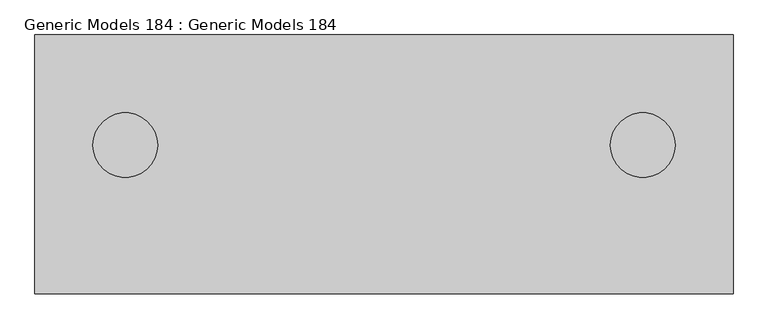
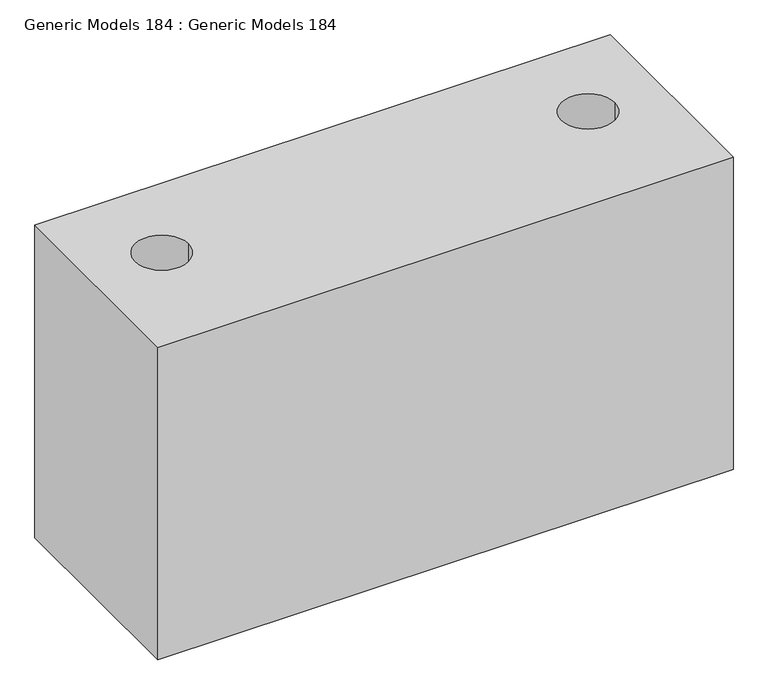
"""IFC4 building model written with IfcOpenShell, lengths in millimetres: proxy geometry, Generic Models 184 : Generic Models 184."""

import ifcopenshell
import ifcopenshell.guid

model = None  # the IFC model being written
_history = None  # IfcOwnerHistory: only IFC2X3 demands one
_inside = {}  # id of a spatial element -> (the spatial element, [elements in it])
_under = {}  # id of a project, library or spatial element -> (it, [spatial elements below it])
_declared = {}  # id of a project -> (the project, [libraries it declares])
_typed = {}  # id of a type object -> (the type object, [elements of that type])
_made_of = {}  # id of a material, layer set ... -> (it, [elements and type objects made of it])


def new_model(schema):
    """Start an empty IFC model of exactly this schema.

    Asked for "IFC4X3", IfcOpenShell would pick the latest addendum, in which some entities
    have other attributes; the version numbers below select the first issue.
    IFC2X3 requires an IfcOwnerHistory on every rooted entity: one is made here for all.
    """
    global model, _history
    if schema == "IFC4X3":
        model = ifcopenshell.file(schema_version=(4, 3, 0, 0))
    else:
        model = ifcopenshell.file(schema=schema)
    _inside.clear()
    _under.clear()
    _declared.clear()
    _typed.clear()
    _made_of.clear()
    _history = None
    if model.schema == "IFC2X3":
        org = make("IfcOrganization", Name="unknown")
        user = make(
            "IfcPersonAndOrganization",
            ThePerson=make("IfcPerson", FamilyName="unknown"),
            TheOrganization=org,
        )
        app = make(
            "IfcApplication",
            ApplicationDeveloper=org,
            Version="unknown",
            ApplicationFullName="unknown",
            ApplicationIdentifier="unknown",
        )
        _history = make(
            "IfcOwnerHistory",
            OwningUser=user,
            OwningApplication=app,
            ChangeAction="ADDED",
            CreationDate=0,
        )
    return model


def make(cls, **values):
    """One entity of the class cls with the attributes given. An attribute that is None is left unset."""
    return model.create_entity(
        cls, **{name: value for name, value in values.items() if value is not None}
    )


def rooted(cls, **values):
    """An entity with a GlobalId (a new one), such as an element, a storey or a relation."""
    return make(cls, GlobalId=ifcopenshell.guid.new(), OwnerHistory=_history, **values)


def si_unit(unit_type, name, prefix=None):
    """IfcSIUnit, for example si_unit("LENGTHUNIT", "METRE", prefix="MILLI")."""
    return make("IfcSIUnit", UnitType=unit_type, Prefix=prefix, Name=name)


def assignment(units):
    """IfcUnitAssignment: the units of a project."""
    return None if units is None else make("IfcUnitAssignment", Units=units)


def point(xyz):
    """IfcCartesianPoint."""
    return None if xyz is None else make("IfcCartesianPoint", Coordinates=xyz)


def direction(xyz):
    """IfcDirection."""
    return None if xyz is None else make("IfcDirection", DirectionRatios=xyz)


def frame(location, z_axis=None, x_axis=None):
    """IfcAxis2Placement3D, a coordinate frame: its origin and axes. An axis left out is left unset."""
    return make(
        "IfcAxis2Placement3D",
        Location=point(location),
        Axis=direction(z_axis),
        RefDirection=direction(x_axis),
    )


def origin():
    """The frame at (0, 0, 0) with its axes left unset."""
    return frame((0.0, 0.0, 0.0))


def place(relative_to, where):
    """IfcLocalPlacement: puts the frame where relative to a parent placement (None: the world)."""
    return make(
        "IfcLocalPlacement", PlacementRelTo=relative_to, RelativePlacement=where
    )


def context(
    kind, dimensions, precision=None, world=None, true_north=None, identifier=None
):
    """IfcGeometricRepresentationContext, for example the 3D "Model" context."""
    return make(
        "IfcGeometricRepresentationContext",
        ContextIdentifier=identifier,
        ContextType=kind,
        CoordinateSpaceDimension=dimensions,
        Precision=precision,
        WorldCoordinateSystem=world,
        TrueNorth=true_north,
    )


def project(units=None, contexts=None):
    """IfcProject with its units and contexts."""
    return rooted(
        "IfcProject",
        Name="project",
        RepresentationContexts=contexts,
        UnitsInContext=assignment(units),
    )


def spatial(cls, under=None, at=None, **own):
    """A site, building, storey or space (cls), placed at a placement, below another one or the project."""
    s = rooted(cls, ObjectPlacement=at, **own)
    if under is not None:
        _under.setdefault(under.id(), (under, []))[1].append(s)
    return s


def polyline(points):
    """IfcPolyline through the points."""
    return make("IfcPolyline", Points=[point(p) for p in points])


def circle_curve(where, radius):
    """IfcCircle in the frame where."""
    return make("IfcCircle", Position=where, Radius=radius)


def shape(context_of_items, identifier, shape_type, items):
    """IfcShapeRepresentation: the items that make up one representation, for example the "Body"."""
    return make(
        "IfcShapeRepresentation",
        ContextOfItems=context_of_items,
        RepresentationIdentifier=identifier,
        RepresentationType=shape_type,
        Items=items,
    )


def source(mapping_origin, context_of_items, identifier, shape_type, items):
    """IfcRepresentationMap: a shape defined once, which mapped items show again and again."""
    return make(
        "IfcRepresentationMap",
        MappingOrigin=mapping_origin,
        MappedRepresentation=shape(context_of_items, identifier, shape_type, items),
    )


def transform(
    local_origin,
    x_axis=None,
    y_axis=None,
    z_axis=None,
    scale=None,
    scale2=None,
    scale3=None,
    uniform=True,
):
    """IfcCartesianTransformationOperator3D, or its non-uniform kind. x_axis, y_axis, z_axis: its Axis1, 2, 3."""
    if uniform:
        return make(
            "IfcCartesianTransformationOperator3D",
            Axis1=direction(x_axis),
            Axis2=direction(y_axis),
            LocalOrigin=point(local_origin),
            Scale=scale,
            Axis3=direction(z_axis),
        )
    return make(
        "IfcCartesianTransformationOperator3DnonUniform",
        Axis1=direction(x_axis),
        Axis2=direction(y_axis),
        LocalOrigin=point(local_origin),
        Scale=scale,
        Axis3=direction(z_axis),
        Scale2=scale2,
        Scale3=scale3,
    )


def mapped(mapping_source, mapping_target):
    """IfcMappedItem: shows the shape of a source again, moved by a transform."""
    return make(
        "IfcMappedItem", MappingSource=mapping_source, MappingTarget=mapping_target
    )


def made_of(thing, what):
    """Note that an element or type object is made of a material, layer set ...; save() writes the relation."""
    if what is not None:
        _made_of.setdefault(what.id(), (what, []))[1].append(thing)
    return thing


def element(
    cls,
    number,
    at=None,
    inside=None,
    cuts=None,
    type_object=None,
    material=None,
    context=None,
    identifier="Body",
    shape_type=None,
    held_by="IfcProductDefinitionShape",
    body=None,
    shapes=None,
    **own,
):
    """One element of the class cls, such as IfcWall. Its Tag is "e" and its number.

    at: its placement. inside: the storey or other place that contains it. cuts: it is an
    opening in that element (IfcRelVoidsElement). A single representation is given by context,
    identifier, shape_type and body (its items); several are given by shapes. held_by: the class
    of the entity that holds the representations. save() writes the other relations.
    """
    e = rooted(cls, Tag="e%d" % number, ObjectPlacement=at, **own)
    if body is not None:
        shapes = [shape(context, identifier, shape_type, body)]
    if shapes is not None:
        e.Representation = make(held_by, Representations=shapes)
    if inside is not None:
        _inside.setdefault(inside.id(), (inside, []))[1].append(e)
    if cuts is not None:
        rooted(
            "IfcRelVoidsElement", RelatingBuildingElement=cuts, RelatedOpeningElement=e
        )
    if type_object is not None:
        _typed.setdefault(type_object.id(), (type_object, []))[1].append(e)
    return made_of(e, material)


def aggregate(whole, parts):
    """IfcRelAggregates: a whole, such as a stair, and the parts it consists of."""
    return rooted("IfcRelAggregates", RelatingObject=whole, RelatedObjects=parts)


def save(model, path):
    """Write the relations noted so far, then the file.

    IfcRelAggregates (storeys below a building ...), IfcRelContainedInSpatialStructure (elements
    in a storey), IfcRelDefinesByType, IfcRelAssociatesMaterial and IfcRelDeclares: one each for
    every whole, place, type object, material and project.
    """
    for whole, parts in _under.values():
        aggregate(whole, parts)
    for where, things in _inside.values():
        rooted(
            "IfcRelContainedInSpatialStructure",
            RelatedElements=things,
            RelatingStructure=where,
        )
    for kind, things in _typed.values():
        rooted("IfcRelDefinesByType", RelatedObjects=things, RelatingType=kind)
    for what, things in _made_of.values():
        rooted("IfcRelAssociatesMaterial", RelatedObjects=things, RelatingMaterial=what)
    for by, libraries in _declared.values():
        rooted("IfcRelDeclares", RelatingContext=by, RelatedDefinitions=libraries)
    model.write(path)


def plane_surface(at):
    """IfcPlane: the flat surface through the origin of the frame at, square to its z axis."""
    return make("IfcPlane", Position=at)


def revolved_surface(curve, axis_point, axis_direction):
    """IfcSurfaceOfRevolution: the curve turned about the line through axis_point along axis_direction."""
    return make(
        "IfcSurfaceOfRevolution",
        SweptCurve=make("IfcArbitraryOpenProfileDef", ProfileType="CURVE", Curve=curve),
        AxisPosition=make("IfcAxis1Placement", Location=point(axis_point), Axis=direction(axis_direction)),
    )


def advanced_brep(points, edges, surfaces, faces):
    """IfcAdvancedBrep: a solid bounded by faces that lie on surfaces and meet in shared edges.

    An edge is (start, end): straight between two places in points (the first is 0);
    or (start, end, curve); or (start, end, curve, False) where it runs against its curve.
    A face is (place in surfaces, loops), or (place, loops, False) where it looks against
    its surface's normal. A loop lists edges by number (the first is 1), with a minus sign
    where the edge is run from its end to its start. The first loop is the outer one.
    """
    corners = [point(p) for p in points]
    vertices = [make("IfcVertexPoint", VertexGeometry=c) for c in corners]
    made = []
    for start, end, *more in edges:
        made.append(
            make(
                "IfcEdgeCurve",
                EdgeStart=vertices[start],
                EdgeEnd=vertices[end],
                EdgeGeometry=more[0] if more else make("IfcPolyline", Points=[corners[start], corners[end]]),
                SameSense=more[1] if len(more) > 1 else True,
            )
        )
    hull = []
    for where, loops, *sense in faces:
        bounds = []
        for j, loop in enumerate(loops):
            ring = [make("IfcOrientedEdge", EdgeElement=made[abs(k) - 1], Orientation=k > 0) for k in loop]
            bounds.append(
                make(
                    "IfcFaceOuterBound" if j == 0 else "IfcFaceBound",
                    Bound=make("IfcEdgeLoop", EdgeList=ring),
                    Orientation=True,
                )
            )
        hull.append(make("IfcAdvancedFace", Bounds=bounds, FaceSurface=surfaces[where], SameSense=sense[0] if sense else True))
    return make("IfcAdvancedBrep", Outer=make("IfcClosedShell", CfsFaces=hull))


def generic_models_184_generic_models_184_067f22a4(model_context):
    return source(origin(), model_context, "Body", "AdvancedBrep", [
        advanced_brep(
        [(57021.4125, 977.9, -23.9117188), (53732.1125, 977.9, -23.9117188), (53732.1125, -241.3, -23.9117188), (57021.4125, -241.3, -23.9117188), (56443.5625, 458.7875, -23.9117188), (56748.3625, 458.7875, -23.9117188), (54005.1625, 458.7875, -23.9117188), (54309.9625, 458.7875, -23.9117188), (57021.4125, 977.9, -1915.3720904), (57021.4125, -241.3, -1915.3720904), (53732.1125, -241.3, -1915.3720904), (53732.1125, 977.9, -1915.3720904), (56443.5625, 458.7875, -1219.2), (56748.3625, 458.7875, -1219.2), (54005.1625, 458.7875, -1219.2), (54309.9625, 458.7875, -1219.2)],
        [
            (0, 1),
            (1, 2),
            (2, 3),
            (3, 0),
            (4, 5, circle_curve(frame((56595.9625, 458.7875, -23.9117188), z_axis=(0.0, 0.0, -1.0), x_axis=(1.0, 0.0, 0.0)), 152.4)),
            (5, 4, circle_curve(frame((56595.9625, 458.7875, -23.9117188), z_axis=(0.0, 0.0, -1.0), x_axis=(1.0, 0.0, 0.0)), 152.4)),
            (6, 7, circle_curve(frame((54157.5625, 458.7875, -23.9117188), z_axis=(0.0, 0.0, -1.0), x_axis=(1.0, 0.0, 0.0)), 152.4)),
            (7, 6, circle_curve(frame((54157.5625, 458.7875, -23.9117188), z_axis=(0.0, 0.0, -1.0), x_axis=(1.0, 0.0, 0.0)), 152.4)),
            (8, 9),
            (9, 10),
            (10, 11),
            (11, 8),
            (0, 8),
            (11, 1),
            (10, 2),
            (9, 3),
            (12, 13, circle_curve(frame((56595.9625, 458.7875, -1219.2), z_axis=(0.0, 0.0, 1.0), x_axis=(1.0, 0.0, 0.0)), 152.4)),
            (13, 12, circle_curve(frame((56595.9625, 458.7875, -1219.2), z_axis=(0.0, 0.0, 1.0), x_axis=(1.0, 0.0, 0.0)), 152.4)),
            (14, 15, circle_curve(frame((54157.5625, 458.7875, -1219.2), z_axis=(0.0, 0.0, 1.0), x_axis=(1.0, 0.0, 0.0)), 152.4)),
            (15, 14, circle_curve(frame((54157.5625, 458.7875, -1219.2), z_axis=(0.0, 0.0, 1.0), x_axis=(1.0, 0.0, 0.0)), 152.4)),
            (13, 5),
            (4, 12),
            (15, 7),
            (6, 14),
        ],
        [
            plane_surface(frame((53732.1125, 977.9, -23.9117188), z_axis=(0.0, 0.0, 1.0), x_axis=(-1.0, 0.0, 0.0))),
            plane_surface(frame((53732.1125, 977.9, -1915.3720904), z_axis=(0.0, 0.0, -1.0), x_axis=(1.0, 0.0, 0.0))),
            plane_surface(frame((57021.4125, 977.9, -23.9117188), z_axis=(0.0, 1.0, 0.0), x_axis=(0.0, 0.0, -1.0))),
            plane_surface(frame((53732.1125, 977.9, -23.9117188), z_axis=(-1.0, 0.0, 0.0), x_axis=(0.0, 0.0, -1.0))),
            plane_surface(frame((53732.1125, -241.3, -23.9117188), z_axis=(0.0, -1.0, 0.0), x_axis=(0.0, 0.0, -1.0))),
            plane_surface(frame((57021.4125, -241.3, -23.9117188), z_axis=(1.0, 0.0, 0.0), x_axis=(0.0, 0.0, -1.0))),
            plane_surface(frame((56748.3625, 458.7875, -1219.2), z_axis=(0.0, 0.0, 1.0), x_axis=(0.0, -1.0, 0.0))),
            revolved_surface(polyline([(56748.3625, 458.7875, -23.911718800000017), (56748.3625, 458.7875, -1219.2)]), (56595.9625, 458.7875, -1219.2), (0.0, 0.0, 1.0)),
            revolved_surface(polyline([(54309.9625, 458.7875, -23.9117188), (54309.9625, 458.7875, -1219.2)]), (54157.5625, 458.7875, 0.0), (0.0, 0.0, 1.0)),
        ],
        [
            (0, [[1, 2, 3, 4], [5, 6], [7, 8]]),
            (1, [[9, 10, 11, 12]]),
            (2, [[-1, 13, -12, 14]]),
            (3, [[-2, -14, -11, 15]]),
            (4, [[-3, -15, -10, 16]]),
            (5, [[-4, -16, -9, -13]]),
            (6, [[17, 18]]),
            (6, [[19, 20]]),
            (7, [[-18, 21, -5, 22]]),
            (7, [[-17, -22, -6, -21]]),
            (8, [[-20, 23, -7, 24]]),
            (8, [[-19, -24, -8, -23]]),
        ],
    ),
    ])


if __name__ == "__main__":
    model = new_model("IFC4")
    model_context = context("Model", 3, world=origin())
    ifc_project = project(units=[si_unit("LENGTHUNIT", "METRE", prefix="MILLI")], contexts=[model_context])
    site = spatial("IfcSite", under=ifc_project)
    building = spatial("IfcBuilding", under=site)
    placement = place(None, origin())
    generic_models_184_generic_models_184_shape = generic_models_184_generic_models_184_067f22a4(model_context)
    element("IfcBuildingElementProxy", 1, Name="Generic Models 184 : Generic Models 184", ObjectType="Generic Models 184 : Generic Models 184", at=placement, inside=building, context=model_context, shape_type="MappedRepresentation", body=[
        mapped(generic_models_184_generic_models_184_shape, transform((0.0, 0.0, 0.0), x_axis=(1.0, 0.0, 0.0), y_axis=(0.0, 1.0, 0.0), z_axis=(0.0, 0.0, 1.0))),
    ])
    save(model, "model.ifc")

# Revit data of these elements
# Element 1 (IfcBuildingElementProxy, "Generic Models 184 : Generic Models 184")
#   Materials on its faces: "GRADE"
# Materials
#   "GRADE": class "Generic", colour RGB 255 255 255, transparency 0, Description = "Soil", Cost = 0
